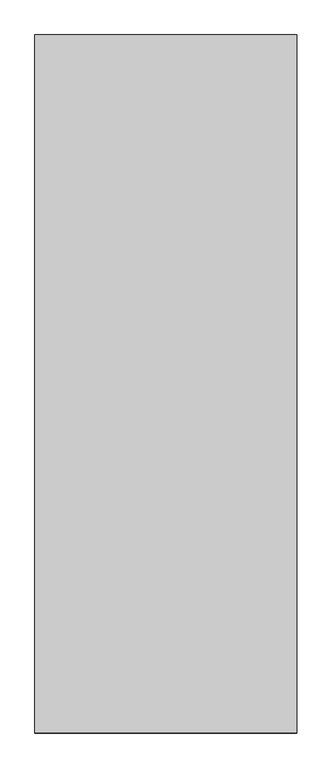
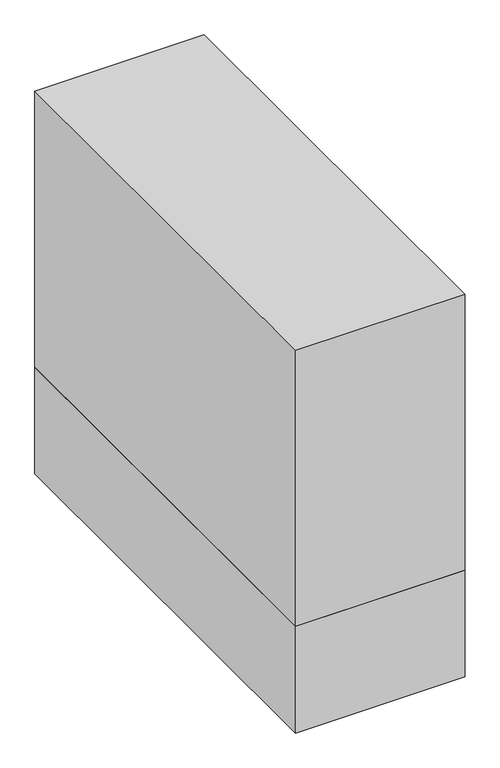
"""IFC4 building model written with IfcOpenShell, lengths in millimetres: furniture geometry, Monument sign1 : Monument sign."""

import ifcopenshell
import ifcopenshell.guid

model = None  # the IFC model being written
_history = None  # IfcOwnerHistory: only IFC2X3 demands one
_inside = {}  # id of a spatial element -> (the spatial element, [elements in it])
_under = {}  # id of a project, library or spatial element -> (it, [spatial elements below it])
_declared = {}  # id of a project -> (the project, [libraries it declares])
_typed = {}  # id of a type object -> (the type object, [elements of that type])
_made_of = {}  # id of a material, layer set ... -> (it, [elements and type objects made of it])


def new_model(schema):
    """Start an empty IFC model of exactly this schema.

    Asked for "IFC4X3", IfcOpenShell would pick the latest addendum, in which some entities
    have other attributes; the version numbers below select the first issue.
    IFC2X3 requires an IfcOwnerHistory on every rooted entity: one is made here for all.
    """
    global model, _history
    if schema == "IFC4X3":
        model = ifcopenshell.file(schema_version=(4, 3, 0, 0))
    else:
        model = ifcopenshell.file(schema=schema)
    _inside.clear()
    _under.clear()
    _declared.clear()
    _typed.clear()
    _made_of.clear()
    _history = None
    if model.schema == "IFC2X3":
        org = make("IfcOrganization", Name="unknown")
        user = make(
            "IfcPersonAndOrganization",
            ThePerson=make("IfcPerson", FamilyName="unknown"),
            TheOrganization=org,
        )
        app = make(
            "IfcApplication",
            ApplicationDeveloper=org,
            Version="unknown",
            ApplicationFullName="unknown",
            ApplicationIdentifier="unknown",
        )
        _history = make(
            "IfcOwnerHistory",
            OwningUser=user,
            OwningApplication=app,
            ChangeAction="ADDED",
            CreationDate=0,
        )
    return model


def make(cls, **values):
    """One entity of the class cls with the attributes given. An attribute that is None is left unset."""
    return model.create_entity(
        cls, **{name: value for name, value in values.items() if value is not None}
    )


def rooted(cls, **values):
    """An entity with a GlobalId (a new one), such as an element, a storey or a relation."""
    return make(cls, GlobalId=ifcopenshell.guid.new(), OwnerHistory=_history, **values)


def si_unit(unit_type, name, prefix=None):
    """IfcSIUnit, for example si_unit("LENGTHUNIT", "METRE", prefix="MILLI")."""
    return make("IfcSIUnit", UnitType=unit_type, Prefix=prefix, Name=name)


def assignment(units):
    """IfcUnitAssignment: the units of a project."""
    return None if units is None else make("IfcUnitAssignment", Units=units)


def point(xyz):
    """IfcCartesianPoint."""
    return None if xyz is None else make("IfcCartesianPoint", Coordinates=xyz)


def direction(xyz):
    """IfcDirection."""
    return None if xyz is None else make("IfcDirection", DirectionRatios=xyz)


def frame(location, z_axis=None, x_axis=None):
    """IfcAxis2Placement3D, a coordinate frame: its origin and axes. An axis left out is left unset."""
    return make(
        "IfcAxis2Placement3D",
        Location=point(location),
        Axis=direction(z_axis),
        RefDirection=direction(x_axis),
    )


def origin():
    """The frame at (0, 0, 0) with its axes left unset."""
    return frame((0.0, 0.0, 0.0))


def place(relative_to, where):
    """IfcLocalPlacement: puts the frame where relative to a parent placement (None: the world)."""
    return make(
        "IfcLocalPlacement", PlacementRelTo=relative_to, RelativePlacement=where
    )


def context(
    kind, dimensions, precision=None, world=None, true_north=None, identifier=None
):
    """IfcGeometricRepresentationContext, for example the 3D "Model" context."""
    return make(
        "IfcGeometricRepresentationContext",
        ContextIdentifier=identifier,
        ContextType=kind,
        CoordinateSpaceDimension=dimensions,
        Precision=precision,
        WorldCoordinateSystem=world,
        TrueNorth=true_north,
    )


def project(units=None, contexts=None):
    """IfcProject with its units and contexts."""
    return rooted(
        "IfcProject",
        Name="project",
        RepresentationContexts=contexts,
        UnitsInContext=assignment(units),
    )


def spatial(cls, under=None, at=None, **own):
    """A site, building, storey or space (cls), placed at a placement, below another one or the project."""
    s = rooted(cls, ObjectPlacement=at, **own)
    if under is not None:
        _under.setdefault(under.id(), (under, []))[1].append(s)
    return s


def polyline(points):
    """IfcPolyline through the points."""
    return make("IfcPolyline", Points=[point(p) for p in points])


def outline(outer, holes=None, kind="AREA"):
    """IfcArbitraryClosedProfileDef: a profile drawn as a closed curve; with holes, ...WithVoids."""
    if holes is None:
        return make("IfcArbitraryClosedProfileDef", ProfileType=kind, OuterCurve=outer)
    return make(
        "IfcArbitraryProfileDefWithVoids",
        ProfileType=kind,
        OuterCurve=outer,
        InnerCurves=holes,
    )


def extrude(swept, where, along, depth):
    """IfcExtrudedAreaSolid: the profile swept, set in the frame where, extruded along a direction by depth."""
    return make(
        "IfcExtrudedAreaSolid",
        SweptArea=swept,
        Position=where,
        ExtrudedDirection=direction(along),
        Depth=depth,
    )


def shape(context_of_items, identifier, shape_type, items):
    """IfcShapeRepresentation: the items that make up one representation, for example the "Body"."""
    return make(
        "IfcShapeRepresentation",
        ContextOfItems=context_of_items,
        RepresentationIdentifier=identifier,
        RepresentationType=shape_type,
        Items=items,
    )


def source(mapping_origin, context_of_items, identifier, shape_type, items):
    """IfcRepresentationMap: a shape defined once, which mapped items show again and again."""
    return make(
        "IfcRepresentationMap",
        MappingOrigin=mapping_origin,
        MappedRepresentation=shape(context_of_items, identifier, shape_type, items),
    )


def transform(
    local_origin,
    x_axis=None,
    y_axis=None,
    z_axis=None,
    scale=None,
    scale2=None,
    scale3=None,
    uniform=True,
):
    """IfcCartesianTransformationOperator3D, or its non-uniform kind. x_axis, y_axis, z_axis: its Axis1, 2, 3."""
    if uniform:
        return make(
            "IfcCartesianTransformationOperator3D",
            Axis1=direction(x_axis),
            Axis2=direction(y_axis),
            LocalOrigin=point(local_origin),
            Scale=scale,
            Axis3=direction(z_axis),
        )
    return make(
        "IfcCartesianTransformationOperator3DnonUniform",
        Axis1=direction(x_axis),
        Axis2=direction(y_axis),
        LocalOrigin=point(local_origin),
        Scale=scale,
        Axis3=direction(z_axis),
        Scale2=scale2,
        Scale3=scale3,
    )


def mapped(mapping_source, mapping_target):
    """IfcMappedItem: shows the shape of a source again, moved by a transform."""
    return make(
        "IfcMappedItem", MappingSource=mapping_source, MappingTarget=mapping_target
    )


def made_of(thing, what):
    """Note that an element or type object is made of a material, layer set ...; save() writes the relation."""
    if what is not None:
        _made_of.setdefault(what.id(), (what, []))[1].append(thing)
    return thing


def element(
    cls,
    number,
    at=None,
    inside=None,
    cuts=None,
    type_object=None,
    material=None,
    context=None,
    identifier="Body",
    shape_type=None,
    held_by="IfcProductDefinitionShape",
    body=None,
    shapes=None,
    **own,
):
    """One element of the class cls, such as IfcWall. Its Tag is "e" and its number.

    at: its placement. inside: the storey or other place that contains it. cuts: it is an
    opening in that element (IfcRelVoidsElement). A single representation is given by context,
    identifier, shape_type and body (its items); several are given by shapes. held_by: the class
    of the entity that holds the representations. save() writes the other relations.
    """
    e = rooted(cls, Tag="e%d" % number, ObjectPlacement=at, **own)
    if body is not None:
        shapes = [shape(context, identifier, shape_type, body)]
    if shapes is not None:
        e.Representation = make(held_by, Representations=shapes)
    if inside is not None:
        _inside.setdefault(inside.id(), (inside, []))[1].append(e)
    if cuts is not None:
        rooted(
            "IfcRelVoidsElement", RelatingBuildingElement=cuts, RelatedOpeningElement=e
        )
    if type_object is not None:
        _typed.setdefault(type_object.id(), (type_object, []))[1].append(e)
    return made_of(e, material)


def aggregate(whole, parts):
    """IfcRelAggregates: a whole, such as a stair, and the parts it consists of."""
    return rooted("IfcRelAggregates", RelatingObject=whole, RelatedObjects=parts)


def save(model, path):
    """Write the relations noted so far, then the file.

    IfcRelAggregates (storeys below a building ...), IfcRelContainedInSpatialStructure (elements
    in a storey), IfcRelDefinesByType, IfcRelAssociatesMaterial and IfcRelDeclares: one each for
    every whole, place, type object, material and project.
    """
    for whole, parts in _under.values():
        aggregate(whole, parts)
    for where, things in _inside.values():
        rooted(
            "IfcRelContainedInSpatialStructure",
            RelatedElements=things,
            RelatingStructure=where,
        )
    for kind, things in _typed.values():
        rooted("IfcRelDefinesByType", RelatedObjects=things, RelatingType=kind)
    for what, things in _made_of.values():
        rooted("IfcRelAssociatesMaterial", RelatedObjects=things, RelatingMaterial=what)
    for by, libraries in _declared.values():
        rooted("IfcRelDeclares", RelatingContext=by, RelatedDefinitions=libraries)
    model.write(path)


def furniture_285fd19a(model_context):
    return source(origin(), model_context, "Body", "SweptSolid", [
        extrude(outline(polyline([(-56111.2091849, 290442.3451888), (-56111.2091849, 292880.7451888), (-55196.8091849, 292880.7451888), (-55196.8091849, 290442.3451888), (-56111.2091849, 290442.3451888)])), frame((0.0, 0.0, -762.0), z_axis=(0.0, 0.0, 1.0), x_axis=(1.0, 0.0, 0.0)), (0.0, 0.0, 1.0), 1574.8),
        extrude(outline(polyline([(-56111.2091849, 292880.7451888), (-55196.8091849, 292880.7451888), (-55196.8091849, 290442.3451888), (-56111.2091849, 290442.3451888), (-56111.2091849, 292880.7451888)])), frame((0.0, 0.0, -1371.6), z_axis=(0.0, 0.0, 1.0), x_axis=(1.0, 0.0, 0.0)), (0.0, 0.0, 1.0), 609.6),
    ])


if __name__ == "__main__":
    model = new_model("IFC4")
    model_context = context("Model", 3, world=origin())
    ifc_project = project(units=[si_unit("LENGTHUNIT", "METRE", prefix="MILLI")], contexts=[model_context])
    site = spatial("IfcSite", under=ifc_project)
    building = spatial("IfcBuilding", under=site)
    placement = place(None, origin())
    furniture_shape = furniture_285fd19a(model_context)
    element("IfcFurniture", 1, ObjectType="Monument sign1 : Monument sign", at=placement, inside=building, context=model_context, shape_type="MappedRepresentation", body=[
        mapped(furniture_shape, transform((0.0, 0.0, 0.0), x_axis=(1.0, 0.0, 0.0), y_axis=(0.0, 1.0, 0.0), z_axis=(0.0, 0.0, 1.0))),
    ])
    save(model, "model.ifc")

# Revit data of these elements
# Element 1 (IfcFurniture, "Monument sign1 : Monument sign")
#   Materials on its faces: "COMPOSITE SIDING (WOOD GRAIN) - TO MATCH MAIN BUILDING", "METAL PANEL (DARK BRONZE) - TO MATCH MAIN BUILDING ACCENT METAL"
# Materials
#   "COMPOSITE SIDING (WOOD GRAIN) - TO MATCH MAIN BUILDING": class "Miscellaneous", colour RGB 143 84 44, transparency 0, Cost = 0
#   "METAL PANEL (DARK BRONZE) - TO MATCH MAIN BUILDING ACCENT METAL": class "Generic", colour RGB 88 62 61, transparency 0, Cost = 0
